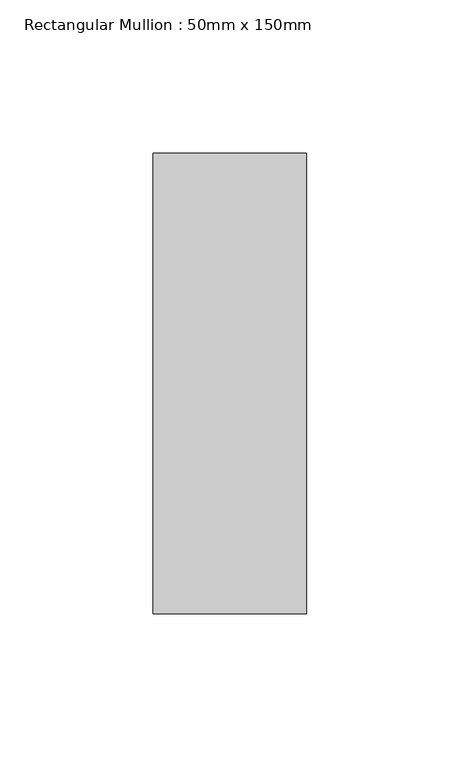
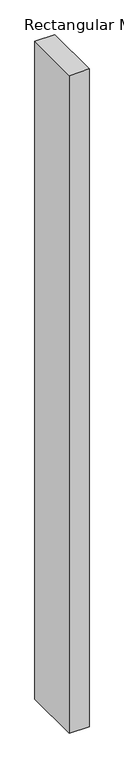
"""IFC4 building model written with IfcOpenShell, lengths in millimetres: member geometry, Rectangular Mullion : 50mm x 150mm."""

from ifc_helpers import new_model, si_unit, frame, origin, place, context, project, spatial, polyline, outline, extrude, source, transform, mapped, element, save


def rectangular_mullion_50mm_x_150mm_4f45a924(model_context):
    return source(origin(), model_context, "Body", "SweptSolid", [
        extrude(outline(polyline([(0.0, 75.0), (0.0, -75.0), (-50.0, -75.0), (-50.0, 75.0), (0.0, 75.0)])), frame((0.0, 0.0, -1755.0000003), z_axis=(0.0, 0.0, 1.0), x_axis=(1.0, 0.0, 0.0)), (0.0, 0.0, 1.0), 1755.0000003),
    ])


if __name__ == "__main__":
    model = new_model("IFC4")
    model_context = context("Model", 3, world=origin())
    ifc_project = project(units=[si_unit("LENGTHUNIT", "METRE", prefix="MILLI")], contexts=[model_context])
    site = spatial("IfcSite", under=ifc_project)
    building = spatial("IfcBuilding", under=site)
    placement = place(None, origin())
    rectangular_mullion_50mm_x_150mm_shape = rectangular_mullion_50mm_x_150mm_4f45a924(model_context)
    element("IfcMember", 1, ObjectType="Rectangular Mullion : 50mm x 150mm", at=placement, inside=building, context=model_context, shape_type="MappedRepresentation", body=[
        mapped(rectangular_mullion_50mm_x_150mm_shape, transform((0.0, 0.0, 0.0), x_axis=(1.0, 0.0, 0.0), y_axis=(0.0, 1.0, 0.0), z_axis=(0.0, 0.0, 1.0))),
    ])
    save(model, "model.ifc")

# Revit data of these elements
# Type "Rectangular Mullion : 50mm x 150mm"
#   built-in parameter 1007304 = 0.492126 (stored number, unit not read)
#   built-in parameter 1007301 = 0.082021 (stored number, unit not read)
#   built-in parameter 1007300 = 0.082021 (stored number, unit not read)
# Element 1 (IfcMember, "Rectangular Mullion : 50mm x 150mm")
#   Materials on its faces: "Aluminum"
# Materials
#   "Aluminum": class "Metal", colour RGB 244 244 244, transparency 0, Description = "Aluminum 6061", Cost = 0
